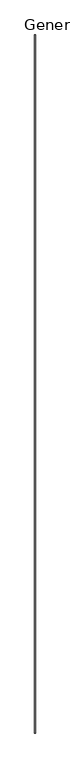
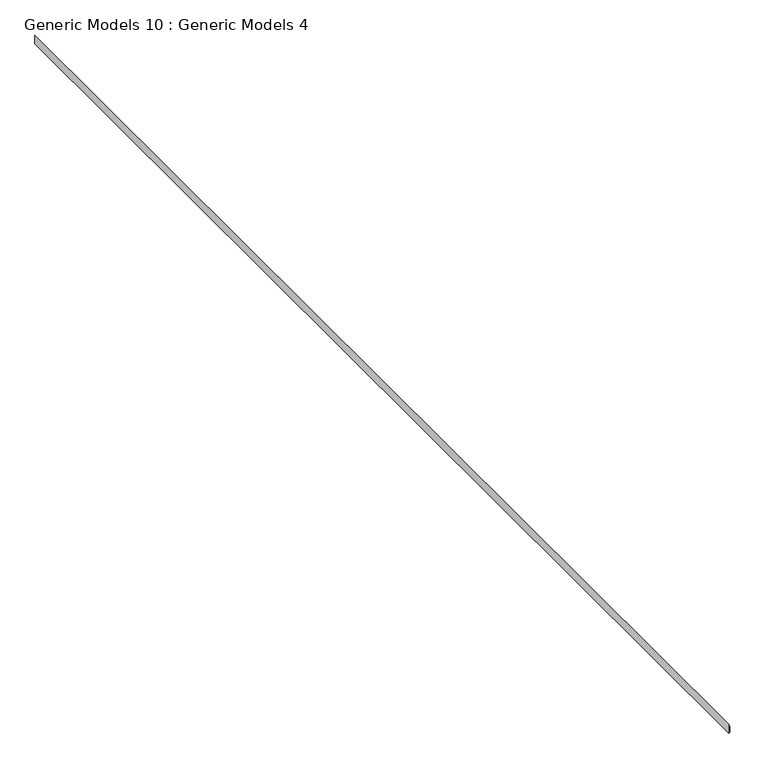
"""IFC4 building model written with IfcOpenShell, lengths in millimetres: proxy geometry, Generic Models 10 : Generic Models 4."""

from ifc_helpers import new_model, si_unit, frame, origin, place, context, project, spatial, polyline, outline, extrude, source, transform, mapped, element, save


def generic_models_10_generic_models_4_dfb9d313(model_context):
    return source(origin(), model_context, "Body", "SweptSolid", [
        extrude(outline(polyline([(126968.835011, 8412.3063704), (127071.2314334, 8412.3063704), (127105.8556439, 8394.5263704), (126963.120011, 8394.5263704), (126968.835011, 8412.3063704)])), frame((0.0, -6864.9230338, 0.0), z_axis=(0.0, 1.0, 0.0), x_axis=(0.0, 0.0, 1.0)), (0.0, 0.0, 1.0), 18643.6),
    ])


if __name__ == "__main__":
    model = new_model("IFC4")
    model_context = context("Model", 3, world=origin())
    ifc_project = project(units=[si_unit("LENGTHUNIT", "METRE", prefix="MILLI")], contexts=[model_context])
    site = spatial("IfcSite", under=ifc_project)
    building = spatial("IfcBuilding", under=site)
    placement = place(None, origin())
    generic_models_10_generic_models_4_shape = generic_models_10_generic_models_4_dfb9d313(model_context)
    element("IfcBuildingElementProxy", 1, Name="Generic Models 10 : Generic Models 4", ObjectType="Generic Models 10 : Generic Models 4", at=placement, inside=building, context=model_context, shape_type="MappedRepresentation", body=[
        mapped(generic_models_10_generic_models_4_shape, transform((0.0, 0.0, 0.0), x_axis=(1.0, 0.0, 0.0), y_axis=(0.0, 1.0, 0.0), z_axis=(0.0, 0.0, 1.0))),
    ])
    save(model, "model.ifc")

# Revit data of these elements
# Element 1 (IfcBuildingElementProxy, "Generic Models 10 : Generic Models 4")
#   Materials on its faces: "_7/8\" SMOOTH TROWEL EXTERIOR STUCCO (COLOR PER OWNER)"
# Materials
#   "_7/8\" SMOOTH TROWEL EXTERIOR STUCCO (COLOR PER OWNER)": class "Generic", colour RGB 233 233 233, transparency 0, Cost = 0
